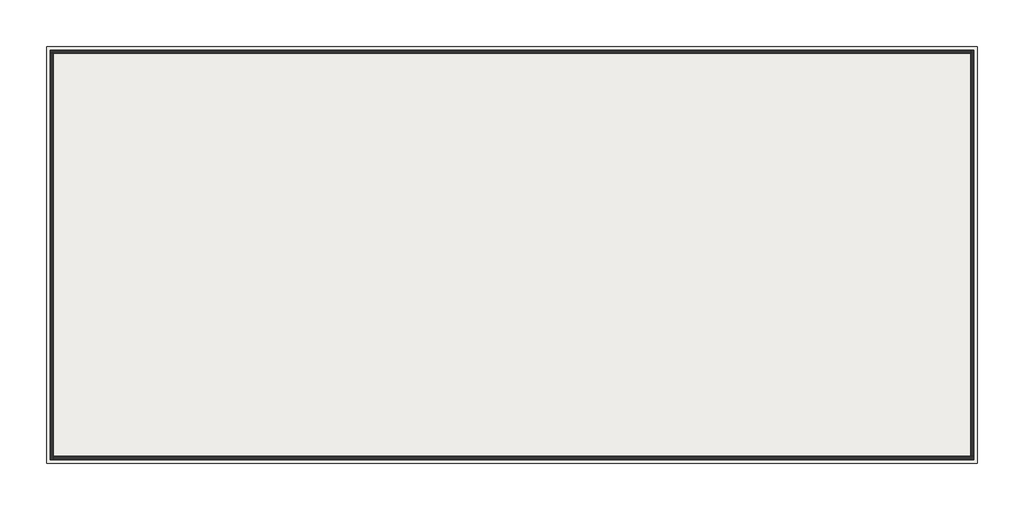
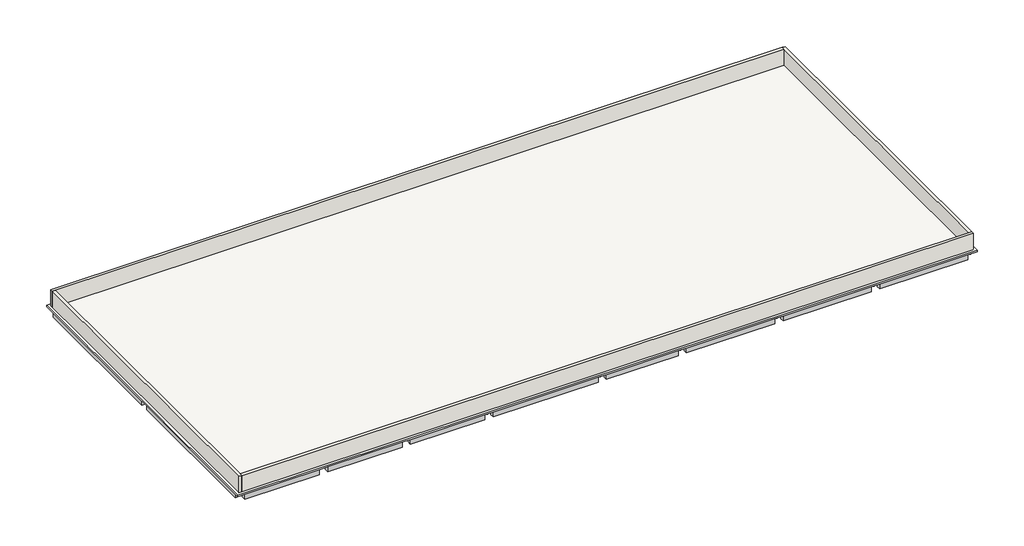
# One storey: 41 beams, 4 walls, 1 roof.
"""IFC4 building model written with IfcOpenShell, lengths in millimetres."""

from ifc_helpers import new_model, si_unit, frame, origin, place, context, project, spatial, polyline, outline, extrude, faceted_brep, element, save

model = new_model("IFC4")

# Units and contexts
model_context = context("Model", 3, world=origin())
ifc_project = project(units=[si_unit("LENGTHUNIT", "METRE", prefix="MILLI")], contexts=[model_context])

# Site, building, storey
site = spatial("IfcSite", under=ifc_project)
building = spatial("IfcBuilding", under=site)
storey = spatial("IfcBuildingStorey", under=building, Name="TOC", Elevation=7649.9618634)

# Beams
placement = place(None, origin())
element("IfcBeam", 1, ObjectType="RC Beam_Rectangular : H_SB_AR_S16_B300xH600", at=placement, inside=storey, context=model_context, shape_type="SweptSolid", body=[
    extrude(outline(polyline([(300.0, 12049.5208589), (300.0, 12349.5208589), (5700.0, 12349.5208589), (5700.0, 12049.5208589), (300.0, 12049.5208589)])), frame((0.0, 0.0, 7049.9618634), z_axis=(0.0, 0.0, 1.0), x_axis=(1.0, 0.0, 0.0)), (0.0, 0.0, 1.0), 499.0),
])
element("IfcBeam", 2, ObjectType="RC Beam_Rectangular : H_SB_AR_S16_B300xH600", at=placement, inside=storey, context=model_context, shape_type="SweptSolid", body=[
    extrude(outline(polyline([(6300.0, 12049.5208589), (6300.0, 12349.5208589), (11700.0, 12349.5208589), (11700.0, 12049.5208589), (6300.0, 12049.5208589)])), frame((0.0, 0.0, 7049.9618634), z_axis=(0.0, 0.0, 1.0), x_axis=(1.0, 0.0, 0.0)), (0.0, 0.0, 1.0), 499.0),
])
element("IfcBeam", 3, ObjectType="RC Beam_Rectangular : H_SB_AR_S16_B300xH600", at=placement, inside=storey, context=model_context, shape_type="SweptSolid", body=[
    extrude(outline(polyline([(12300.0, 12049.5208589), (12300.0, 12349.5208589), (17700.0, 12349.5208589), (17700.0, 12049.5208589), (12300.0, 12049.5208589)])), frame((0.0, 0.0, 7049.9618634), z_axis=(0.0, 0.0, 1.0), x_axis=(1.0, 0.0, 0.0)), (0.0, 0.0, 1.0), 499.0),
])
element("IfcBeam", 4, ObjectType="RC Beam_Rectangular : H_SB_AR_S16_B300xH600", at=placement, inside=storey, context=model_context, shape_type="SweptSolid", body=[
    extrude(outline(polyline([(300.0, 23749.5208589), (300.0, 24049.5208589), (5700.0, 24049.5208589), (5700.0, 23749.5208589), (300.0, 23749.5208589)])), frame((0.0, 0.0, 7049.9618634), z_axis=(0.0, 0.0, 1.0), x_axis=(1.0, 0.0, 0.0)), (0.0, 0.0, 1.0), 499.0),
])
element("IfcBeam", 5, ObjectType="RC Beam_Rectangular : H_SB_AR_S16_B300xH600", at=placement, inside=storey, context=model_context, shape_type="SweptSolid", body=[
    extrude(outline(polyline([(6300.0, 23749.5208589), (6300.0, 24049.5208589), (11700.0, 24049.5208589), (11700.0, 23749.5208589), (6300.0, 23749.5208589)])), frame((0.0, 0.0, 7049.9618634), z_axis=(0.0, 0.0, 1.0), x_axis=(1.0, 0.0, 0.0)), (0.0, 0.0, 1.0), 499.0),
])
element("IfcBeam", 6, ObjectType="RC Beam_Rectangular : H_SB_AR_S16_B300xH600", at=placement, inside=storey, context=model_context, shape_type="SweptSolid", body=[
    extrude(outline(polyline([(12300.0, 23749.5208589), (12300.0, 24049.5208589), (17700.0, 24049.5208589), (17700.0, 23749.5208589), (12300.0, 23749.5208589)])), frame((0.0, 0.0, 7049.9618634), z_axis=(0.0, 0.0, 1.0), x_axis=(1.0, 0.0, 0.0)), (0.0, 0.0, 1.0), 499.0),
])
element("IfcBeam", 7, ObjectType="RC Beam_Rectangular : H_SB_AR_S16_B300xH600", at=placement, inside=storey, context=model_context, shape_type="SweptSolid", body=[
    extrude(outline(polyline([(18300.0, 23749.5208589), (18300.0, 24049.5208589), (25900.0, 24049.5208589), (25900.0, 23749.5208589), (18300.0, 23749.5208589)])), frame((0.0, 0.0, 7049.9618634), z_axis=(0.0, 0.0, 1.0), x_axis=(1.0, 0.0, 0.0)), (0.0, 0.0, 1.0), 499.0),
])
element("IfcBeam", 8, ObjectType="RC Beam_Rectangular : H_SB_AR_S16_B300xH600", at=placement, inside=storey, context=model_context, shape_type="SweptSolid", body=[
    extrude(outline(polyline([(26500.0, 23749.5208589), (26500.0, 24049.5208589), (31700.0, 24049.5208589), (31700.0, 23749.5208589), (26500.0, 23749.5208589)])), frame((0.0, 0.0, 7049.9618634), z_axis=(0.0, 0.0, 1.0), x_axis=(1.0, 0.0, 0.0)), (0.0, 0.0, 1.0), 499.0),
])
element("IfcBeam", 9, ObjectType="RC Beam_Rectangular : H_SB_AR_S16_B300xH600", at=placement, inside=storey, context=model_context, shape_type="SweptSolid", body=[
    extrude(outline(polyline([(32300.0, 23749.5208589), (32300.0, 24049.5208589), (38700.0, 24049.5208589), (38700.0, 23749.5208589), (32300.0, 23749.5208589)])), frame((0.0, 0.0, 7049.9618634), z_axis=(0.0, 0.0, 1.0), x_axis=(1.0, 0.0, 0.0)), (0.0, 0.0, 1.0), 499.0),
])
element("IfcBeam", 10, ObjectType="RC Beam_Rectangular : H_SB_AR_S16_B300xH600", at=placement, inside=storey, context=model_context, shape_type="SweptSolid", body=[
    extrude(outline(polyline([(39300.0, 23749.5208589), (39300.0, 24049.5208589), (45700.0, 24049.5208589), (45700.0, 23749.5208589), (39300.0, 23749.5208589)])), frame((0.0, 0.0, 7049.9618634), z_axis=(0.0, 0.0, 1.0), x_axis=(1.0, 0.0, 0.0)), (0.0, 0.0, 1.0), 499.0),
])
element("IfcBeam", 11, ObjectType="RC Beam_Rectangular : H_SB_AR_S16_B300xH600", at=placement, inside=storey, context=model_context, shape_type="SweptSolid", body=[
    extrude(outline(polyline([(46300.0, 23749.5208589), (46300.0, 24049.5208589), (52700.0, 24049.5208589), (52700.0, 23749.5208589), (46300.0, 23749.5208589)])), frame((0.0, 0.0, 7049.9618634), z_axis=(0.0, 0.0, 1.0), x_axis=(1.0, 0.0, 0.0)), (0.0, 0.0, 1.0), 499.0),
])
element("IfcBeam", 12, ObjectType="RC Beam_Rectangular : H_SB_AR_S16_B300xH600", at=placement, inside=storey, context=model_context, shape_type="SweptSolid", body=[
    extrude(outline(polyline([(26500.0, 8149.5208589), (26500.0, 8449.5208589), (31700.0, 8449.5208589), (31700.0, 8149.5208589), (26500.0, 8149.5208589)])), frame((0.0, 0.0, 7049.9618634), z_axis=(0.0, 0.0, 1.0), x_axis=(1.0, 0.0, 0.0)), (0.0, 0.0, 1.0), 499.0),
])
element("IfcBeam", 13, ObjectType="RC Beam_Rectangular : H_SB_AR_S16_B300xH600", at=placement, inside=storey, context=model_context, shape_type="SweptSolid", body=[
    extrude(outline(polyline([(32300.0, 8149.5208589), (32300.0, 8449.5208589), (38700.0, 8449.5208589), (38700.0, 8149.5208589), (32300.0, 8149.5208589)])), frame((0.0, 0.0, 7049.9618634), z_axis=(0.0, 0.0, 1.0), x_axis=(1.0, 0.0, 0.0)), (0.0, 0.0, 1.0), 499.0),
])
element("IfcBeam", 14, ObjectType="RC Beam_Rectangular : H_SB_AR_S16_B300xH600", at=placement, inside=storey, context=model_context, shape_type="SweptSolid", body=[
    extrude(outline(polyline([(39300.0, 8149.5208589), (39300.0, 8449.5208589), (45700.0, 8449.5208589), (45700.0, 8149.5208589), (39300.0, 8149.5208589)])), frame((0.0, 0.0, 7049.9618634), z_axis=(0.0, 0.0, 1.0), x_axis=(1.0, 0.0, 0.0)), (0.0, 0.0, 1.0), 499.0),
])
element("IfcBeam", 15, ObjectType="RC Beam_Rectangular : H_SB_AR_S16_B300xH600", at=placement, inside=storey, context=model_context, shape_type="SweptSolid", body=[
    extrude(outline(polyline([(46300.0, 8149.5208589), (46300.0, 8449.5208589), (52700.0, 8449.5208589), (52700.0, 8149.5208589), (46300.0, 8149.5208589)])), frame((0.0, 0.0, 7049.9618634), z_axis=(0.0, 0.0, 1.0), x_axis=(1.0, 0.0, 0.0)), (0.0, 0.0, 1.0), 499.0),
])
element("IfcBeam", 16, ObjectType="RC Beam_Rectangular : H_SB_AR_S16_B300xH600", at=placement, inside=storey, context=model_context, shape_type="SweptSolid", body=[
    extrude(outline(polyline([(300.0, 349.5208589), (300.0, 649.5208589), (5700.0, 649.5208589), (5700.0, 349.5208589), (300.0, 349.5208589)])), frame((0.0, 0.0, 7049.9618634), z_axis=(0.0, 0.0, 1.0), x_axis=(1.0, 0.0, 0.0)), (0.0, 0.0, 1.0), 499.0),
])
element("IfcBeam", 17, ObjectType="RC Beam_Rectangular : H_SB_AR_S16_B300xH600", at=placement, inside=storey, context=model_context, shape_type="SweptSolid", body=[
    extrude(outline(polyline([(6300.0, 349.5208589), (6300.0, 649.5208589), (11700.0, 649.5208589), (11700.0, 349.5208589), (6300.0, 349.5208589)])), frame((0.0, 0.0, 7049.9618634), z_axis=(0.0, 0.0, 1.0), x_axis=(1.0, 0.0, 0.0)), (0.0, 0.0, 1.0), 499.0),
])
element("IfcBeam", 18, ObjectType="RC Beam_Rectangular : H_SB_AR_S16_B300xH600", at=placement, inside=storey, context=model_context, shape_type="SweptSolid", body=[
    extrude(outline(polyline([(12300.0, 349.5208589), (12300.0, 649.5208589), (17700.0, 649.5208589), (17700.0, 349.5208589), (12300.0, 349.5208589)])), frame((0.0, 0.0, 7049.9618634), z_axis=(0.0, 0.0, 1.0), x_axis=(1.0, 0.0, 0.0)), (0.0, 0.0, 1.0), 499.0),
])
element("IfcBeam", 19, ObjectType="RC Beam_Rectangular : H_SB_AR_S16_B300xH600", at=placement, inside=storey, context=model_context, shape_type="SweptSolid", body=[
    extrude(outline(polyline([(18300.0, 349.5208589), (18300.0, 649.5208589), (25900.0, 649.5208589), (25900.0, 349.5208589), (18300.0, 349.5208589)])), frame((0.0, 0.0, 7049.9618634), z_axis=(0.0, 0.0, 1.0), x_axis=(1.0, 0.0, 0.0)), (0.0, 0.0, 1.0), 499.0),
])
element("IfcBeam", 20, ObjectType="RC Beam_Rectangular : H_SB_AR_S16_B300xH600", at=placement, inside=storey, context=model_context, shape_type="SweptSolid", body=[
    extrude(outline(polyline([(26500.0, 349.5208589), (26500.0, 649.5208589), (31700.0, 649.5208589), (31700.0, 349.5208589), (26500.0, 349.5208589)])), frame((0.0, 0.0, 7049.9618634), z_axis=(0.0, 0.0, 1.0), x_axis=(1.0, 0.0, 0.0)), (0.0, 0.0, 1.0), 499.0),
])
element("IfcBeam", 21, ObjectType="RC Beam_Rectangular : H_SB_AR_S16_B300xH600", at=placement, inside=storey, context=model_context, shape_type="SweptSolid", body=[
    extrude(outline(polyline([(32300.0, 349.5208589), (32300.0, 649.5208589), (38700.0, 649.5208589), (38700.0, 349.5208589), (32300.0, 349.5208589)])), frame((0.0, 0.0, 7049.9618634), z_axis=(0.0, 0.0, 1.0), x_axis=(1.0, 0.0, 0.0)), (0.0, 0.0, 1.0), 499.0),
])
element("IfcBeam", 22, ObjectType="RC Beam_Rectangular : H_SB_AR_S16_B300xH600", at=placement, inside=storey, context=model_context, shape_type="SweptSolid", body=[
    extrude(outline(polyline([(39300.0, 349.5208589), (39300.0, 649.5208589), (45700.0, 649.5208589), (45700.0, 349.5208589), (39300.0, 349.5208589)])), frame((0.0, 0.0, 7049.9618634), z_axis=(0.0, 0.0, 1.0), x_axis=(1.0, 0.0, 0.0)), (0.0, 0.0, 1.0), 499.0),
])
element("IfcBeam", 23, ObjectType="RC Beam_Rectangular : H_SB_AR_S16_B300xH600", at=placement, inside=storey, context=model_context, shape_type="SweptSolid", body=[
    extrude(outline(polyline([(46300.0, 349.5208589), (46300.0, 649.5208589), (52700.0, 649.5208589), (52700.0, 349.5208589), (46300.0, 349.5208589)])), frame((0.0, 0.0, 7049.9618634), z_axis=(0.0, 0.0, 1.0), x_axis=(1.0, 0.0, 0.0)), (0.0, 0.0, 1.0), 499.0),
])
element("IfcBeam", 24, ObjectType="RC Beam_Rectangular : H_SB_AR_S16_B300xH600", at=placement, inside=storey, context=model_context, shape_type="SweptSolid", body=[
    extrude(outline(polyline([(150.0, 799.5208589), (-150.0, 799.5208589), (-150.0, 11899.5208589), (150.0, 11899.5208589), (150.0, 799.5208589)])), frame((0.0, 0.0, 7049.9618634), z_axis=(0.0, 0.0, 1.0), x_axis=(1.0, 0.0, 0.0)), (0.0, 0.0, 1.0), 499.0),
])
element("IfcBeam", 25, ObjectType="RC Beam_Rectangular : H_SB_AR_S16_B300xH600", at=placement, inside=storey, context=model_context, shape_type="SweptSolid", body=[
    extrude(outline(polyline([(-150.0, 23599.5208589), (150.0, 23599.5208589), (150.0, 12499.5208589), (-150.0, 12499.5208589), (-150.0, 23599.5208589)])), frame((0.0, 0.0, 7049.9618634), z_axis=(0.0, 0.0, 1.0), x_axis=(1.0, 0.0, 0.0)), (0.0, 0.0, 1.0), 499.0),
])
element("IfcBeam", 26, ObjectType="RC Beam_Rectangular : H_SB_AR_S16_B300xH600", at=placement, inside=storey, context=model_context, shape_type="SweptSolid", body=[
    extrude(outline(polyline([(5850.0, 11899.5208589), (6150.0, 11899.5208589), (6150.0, 799.5208589), (5850.0, 799.5208589), (5850.0, 11899.5208589)])), frame((0.0, 0.0, 7049.9618634), z_axis=(0.0, 0.0, 1.0), x_axis=(1.0, 0.0, 0.0)), (0.0, 0.0, 1.0), 499.0),
])
element("IfcBeam", 27, ObjectType="RC Beam_Rectangular : H_SB_AR_S16_B300xH600", at=placement, inside=storey, context=model_context, shape_type="SweptSolid", body=[
    extrude(outline(polyline([(6150.0, 12499.5208589), (5850.0, 12499.5208589), (5850.0, 23599.5208589), (6150.0, 23599.5208589), (6150.0, 12499.5208589)])), frame((0.0, 0.0, 7049.9618634), z_axis=(0.0, 0.0, 1.0), x_axis=(1.0, 0.0, 0.0)), (0.0, 0.0, 1.0), 499.0),
])
element("IfcBeam", 28, ObjectType="RC Beam_Rectangular : H_SB_AR_S16_B300xH600", at=placement, inside=storey, context=model_context, shape_type="SweptSolid", body=[
    extrude(outline(polyline([(11850.0, 11899.5208589), (12150.0, 11899.5208589), (12150.0, 799.5208589), (11850.0, 799.5208589), (11850.0, 11899.5208589)])), frame((0.0, 0.0, 7049.9618634), z_axis=(0.0, 0.0, 1.0), x_axis=(1.0, 0.0, 0.0)), (0.0, 0.0, 1.0), 499.0),
])
element("IfcBeam", 29, ObjectType="RC Beam_Rectangular : H_SB_AR_S16_B300xH600", at=placement, inside=storey, context=model_context, shape_type="SweptSolid", body=[
    extrude(outline(polyline([(12150.0, 12499.5208589), (11850.0, 12499.5208589), (11850.0, 23599.5208589), (12150.0, 23599.5208589), (12150.0, 12499.5208589)])), frame((0.0, 0.0, 7049.9618634), z_axis=(0.0, 0.0, 1.0), x_axis=(1.0, 0.0, 0.0)), (0.0, 0.0, 1.0), 499.0),
])
element("IfcBeam", 30, ObjectType="RC Beam_Rectangular : H_SB_AR_S16_B300xH600", at=placement, inside=storey, context=model_context, shape_type="SweptSolid", body=[
    extrude(outline(polyline([(17850.0, 11899.5208589), (18150.0, 11899.5208589), (18150.0, 799.5208589), (17850.0, 799.5208589), (17850.0, 11899.5208589)])), frame((0.0, 0.0, 7049.9618634), z_axis=(0.0, 0.0, 1.0), x_axis=(1.0, 0.0, 0.0)), (0.0, 0.0, 1.0), 499.0),
])
element("IfcBeam", 31, ObjectType="RC Beam_Rectangular : H_SB_AR_S16_B300xH600", at=placement, inside=storey, context=model_context, shape_type="SweptSolid", body=[
    extrude(outline(polyline([(18150.0, 12499.5208589), (17850.0, 12499.5208589), (17850.0, 23599.5208589), (18150.0, 23599.5208589), (18150.0, 12499.5208589)])), frame((0.0, 0.0, 7049.9618634), z_axis=(0.0, 0.0, 1.0), x_axis=(1.0, 0.0, 0.0)), (0.0, 0.0, 1.0), 499.0),
])
element("IfcBeam", 32, ObjectType="RC Beam_Rectangular : H_SB_AR_S16_B300xH600", at=placement, inside=storey, context=model_context, shape_type="SweptSolid", body=[
    extrude(outline(polyline([(26050.0, 7999.5208589), (26350.0, 7999.5208589), (26350.0, 799.5208589), (26050.0, 799.5208589), (26050.0, 7999.5208589)])), frame((0.0, 0.0, 7049.9618634), z_axis=(0.0, 0.0, 1.0), x_axis=(1.0, 0.0, 0.0)), (0.0, 0.0, 1.0), 499.0),
])
element("IfcBeam", 33, ObjectType="RC Beam_Rectangular : H_SB_AR_S16_B300xH600", at=placement, inside=storey, context=model_context, shape_type="SweptSolid", body=[
    extrude(outline(polyline([(26050.0, 23599.5208589), (26350.0, 23599.5208589), (26350.0, 8599.5208589), (26050.0, 8599.5208589), (26050.0, 23599.5208589)])), frame((0.0, 0.0, 7049.9618634), z_axis=(0.0, 0.0, 1.0), x_axis=(1.0, 0.0, 0.0)), (0.0, 0.0, 1.0), 499.0),
])
element("IfcBeam", 34, ObjectType="RC Beam_Rectangular : H_SB_AR_S16_B300xH600", at=placement, inside=storey, context=model_context, shape_type="SweptSolid", body=[
    extrude(outline(polyline([(31850.0, 7999.5208589), (32150.0, 7999.5208589), (32150.0, 799.5208589), (31850.0, 799.5208589), (31850.0, 7999.5208589)])), frame((0.0, 0.0, 7049.9618634), z_axis=(0.0, 0.0, 1.0), x_axis=(1.0, 0.0, 0.0)), (0.0, 0.0, 1.0), 499.0),
])
element("IfcBeam", 35, ObjectType="RC Beam_Rectangular : H_SB_AR_S16_B300xH600", at=placement, inside=storey, context=model_context, shape_type="SweptSolid", body=[
    extrude(outline(polyline([(31850.0, 23599.5208589), (32150.0, 23599.5208589), (32150.0, 8599.5208589), (31850.0, 8599.5208589), (31850.0, 23599.5208589)])), frame((0.0, 0.0, 7049.9618634), z_axis=(0.0, 0.0, 1.0), x_axis=(1.0, 0.0, 0.0)), (0.0, 0.0, 1.0), 499.0),
])
element("IfcBeam", 36, ObjectType="RC Beam_Rectangular : H_SB_AR_S16_B300xH600", at=placement, inside=storey, context=model_context, shape_type="SweptSolid", body=[
    extrude(outline(polyline([(38850.0, 7999.5208589), (39150.0, 7999.5208589), (39150.0, 799.5208589), (38850.0, 799.5208589), (38850.0, 7999.5208589)])), frame((0.0, 0.0, 7049.9618634), z_axis=(0.0, 0.0, 1.0), x_axis=(1.0, 0.0, 0.0)), (0.0, 0.0, 1.0), 499.0),
])
element("IfcBeam", 37, ObjectType="RC Beam_Rectangular : H_SB_AR_S16_B300xH600", at=placement, inside=storey, context=model_context, shape_type="SweptSolid", body=[
    extrude(outline(polyline([(38850.0, 23599.5208589), (39150.0, 23599.5208589), (39150.0, 8599.5208589), (38850.0, 8599.5208589), (38850.0, 23599.5208589)])), frame((0.0, 0.0, 7049.9618634), z_axis=(0.0, 0.0, 1.0), x_axis=(1.0, 0.0, 0.0)), (0.0, 0.0, 1.0), 499.0),
])
element("IfcBeam", 38, ObjectType="RC Beam_Rectangular : H_SB_AR_S16_B300xH600", at=placement, inside=storey, context=model_context, shape_type="SweptSolid", body=[
    extrude(outline(polyline([(45850.0, 7999.5208589), (46150.0, 7999.5208589), (46150.0, 799.5208589), (45850.0, 799.5208589), (45850.0, 7999.5208589)])), frame((0.0, 0.0, 7049.9618634), z_axis=(0.0, 0.0, 1.0), x_axis=(1.0, 0.0, 0.0)), (0.0, 0.0, 1.0), 499.0),
])
element("IfcBeam", 39, ObjectType="RC Beam_Rectangular : H_SB_AR_S16_B300xH600", at=placement, inside=storey, context=model_context, shape_type="SweptSolid", body=[
    extrude(outline(polyline([(45850.0, 23599.5208589), (46150.0, 23599.5208589), (46150.0, 8599.5208589), (45850.0, 8599.5208589), (45850.0, 23599.5208589)])), frame((0.0, 0.0, 7049.9618634), z_axis=(0.0, 0.0, 1.0), x_axis=(1.0, 0.0, 0.0)), (0.0, 0.0, 1.0), 499.0),
])
element("IfcBeam", 40, ObjectType="RC Beam_Rectangular : H_SB_AR_S16_B300xH600", at=placement, inside=storey, context=model_context, shape_type="SweptSolid", body=[
    extrude(outline(polyline([(53150.0, 799.5208589), (52850.0, 799.5208589), (52850.0, 7999.5208589), (53150.0, 7999.5208589), (53150.0, 799.5208589)])), frame((0.0, 0.0, 7049.9618634), z_axis=(0.0, 0.0, 1.0), x_axis=(1.0, 0.0, 0.0)), (0.0, 0.0, 1.0), 499.0),
])
element("IfcBeam", 41, ObjectType="RC Beam_Rectangular : H_SB_AR_S16_B300xH600", at=placement, inside=storey, context=model_context, shape_type="SweptSolid", body=[
    extrude(outline(polyline([(53150.0, 8599.5208589), (52850.0, 8599.5208589), (52850.0, 23599.5208589), (53150.0, 23599.5208589), (53150.0, 8599.5208589)])), frame((0.0, 0.0, 7049.9618634), z_axis=(0.0, 0.0, 1.0), x_axis=(1.0, 0.0, 0.0)), (0.0, 0.0, 1.0), 499.0),
])

# Roof
element("IfcRoof", 42, ObjectType="H_RF_AR_B06_Memb_XPS_PE_Protective Conc", at=placement, inside=storey, context=model_context, shape_type="Brep", body=[
    faceted_brep([(53300.0, 24199.5208589, 7548.9618634), (53300.0, 23599.5208589, 7548.9618634), (53300.0, 8599.5208589, 7548.9618634), (53300.0, 7999.5208589, 7548.9618634), (53300.0, 799.5208589, 7548.9618634), (53300.0, 199.5208589, 7548.9618634), (52700.0, 199.5208589, 7548.9618634), (46300.0, 199.5208589, 7548.9618634), (45700.0, 199.5208589, 7548.9618634), (39300.0, 199.5208589, 7548.9618634), (38700.0, 199.5208589, 7548.9618634), (32300.0, 199.5208589, 7548.9618634), (31700.0, 199.5208589, 7548.9618634), (26500.0, 199.5208589, 7548.9618634), (25900.0, 199.5208589, 7548.9618634), (18300.0, 199.5208589, 7548.9618634), (17700.0, 199.5208589, 7548.9618634), (12300.0, 199.5208589, 7548.9618634), (11700.0, 199.5208589, 7548.9618634), (6300.0, 199.5208589, 7548.9618634), (5700.0, 199.5208589, 7548.9618634), (300.0, 199.5208589, 7548.9618634), (-300.0, 199.5208589, 7548.9618634), (-300.0, 799.5208589, 7548.9618634), (-300.0, 11899.5208589, 7548.9618634), (-300.0, 12499.5208589, 7548.9618634), (-300.0, 23599.5208589, 7548.9618634), (-300.0, 24199.5208589, 7548.9618634), (300.0, 24199.5208589, 7548.9618634), (5700.0, 24199.5208589, 7548.9618634), (6300.0, 24199.5208589, 7548.9618634), (11700.0, 24199.5208589, 7548.9618634), (12300.0, 24199.5208589, 7548.9618634), (17700.0, 24199.5208589, 7548.9618634), (18300.0, 24199.5208589, 7548.9618634), (25900.0, 24199.5208589, 7548.9618634), (26500.0, 24199.5208589, 7548.9618634), (31700.0, 24199.5208589, 7548.9618634), (32300.0, 24199.5208589, 7548.9618634), (38700.0, 24199.5208589, 7548.9618634), (39300.0, 24199.5208589, 7548.9618634), (45700.0, 24199.5208589, 7548.9618634), (46300.0, 24199.5208589, 7548.9618634), (52700.0, 24199.5208589, 7548.9618634), (53300.0, 199.5208589, 7649.9618634), (53300.0, 24199.5208589, 7649.9618634), (-300.0, 24199.5208589, 7649.9618634), (-300.0, 199.5208589, 7649.9618634)], [[[0, 1, 2, 3, 4, 5, 6, 7, 8, 9, 10, 11, 12, 13, 14, 15, 16, 17, 18, 19, 20, 21, 22, 23, 24, 25, 26, 27, 28, 29, 30, 31, 32, 33, 34, 35, 36, 37, 38, 39, 40, 41, 42, 43]], [[44, 45, 46, 47]], [[45, 44, 5, 4, 3, 2, 1, 0]], [[46, 45, 0, 43, 42, 41, 40, 39, 38, 37, 36, 35, 34, 33, 32, 31, 30, 29, 28, 27]], [[47, 46, 27, 26, 25, 24, 23, 22]], [[44, 47, 22, 21, 20, 19, 18, 17, 16, 15, 14, 13, 12, 11, 10, 9, 8, 7, 6, 5]]]),
])

# Walls
element("IfcWall", 43, ObjectType="H_WA_AR_B02_Ext Wall_RC T200", at=placement, inside=storey, context=model_context, shape_type="Brep", body=[
    faceted_brep([(-100.0, 23799.5208589, 7649.9618634), (100.0, 23799.5208589, 7649.9618634), (52900.0, 23799.5208589, 7649.9618634), (52900.0, 23799.5208589, 8899.9618634), (100.0, 23799.5208589, 8899.9618634), (-100.0, 23799.5208589, 8899.9618634), (-100.0, 23999.5208589, 7649.9618634), (-100.0, 23999.5208589, 8899.9618634), (52900.0, 23999.5208589, 8899.9618634), (52900.0, 23999.5208589, 7649.9618634)], [[[0, 1, 2, 3, 4, 5]], [[6, 7, 8, 9]], [[2, 1, 0, 6, 9]], [[5, 4, 3, 8, 7]], [[0, 5, 7, 6]], [[3, 2, 9, 8]]]),
])
element("IfcWall", 44, ObjectType="H_WA_AR_B02_Ext Wall_RC T200", at=placement, inside=storey, context=model_context, shape_type="Brep", body=[
    faceted_brep([(100.0, 399.5208589, 7649.9618634), (100.0, 599.5208589, 7649.9618634), (100.0, 23799.5208589, 7649.9618634), (100.0, 23799.5208589, 8899.9618634), (100.0, 599.5208589, 8899.9618634), (100.0, 399.5208589, 8899.9618634), (-100.0, 399.5208589, 7649.9618634), (-100.0, 399.5208589, 8899.9618634), (-100.0, 23799.5208589, 8899.9618634), (-100.0, 23799.5208589, 7649.9618634)], [[[0, 1, 2, 3, 4, 5]], [[6, 7, 8, 9]], [[2, 1, 0, 6, 9]], [[5, 4, 3, 8, 7]], [[0, 5, 7, 6]], [[3, 2, 9, 8]]]),
])
element("IfcWall", 45, ObjectType="H_WA_AR_B02_Ext Wall_RC T200", at=placement, inside=storey, context=model_context, shape_type="Brep", body=[
    faceted_brep([(53100.0, 599.5208589, 7649.9618634), (52900.0, 599.5208589, 7649.9618634), (100.0, 599.5208589, 7649.9618634), (100.0, 599.5208589, 8899.9618634), (52900.0, 599.5208589, 8899.9618634), (53100.0, 599.5208589, 8899.9618634), (53100.0, 399.5208589, 7649.9618634), (53100.0, 399.5208589, 8899.9618634), (100.0, 399.5208589, 8899.9618634), (100.0, 399.5208589, 7649.9618634)], [[[0, 1, 2, 3, 4, 5]], [[6, 7, 8, 9]], [[2, 1, 0, 6, 9]], [[5, 4, 3, 8, 7]], [[0, 5, 7, 6]], [[3, 2, 9, 8]]]),
])
element("IfcWall", 46, ObjectType="H_WA_AR_B02_Ext Wall_RC T200", at=placement, inside=storey, context=model_context, shape_type="Brep", body=[
    faceted_brep([(52900.0, 23999.5208589, 7649.9618634), (52900.0, 23799.5208589, 7649.9618634), (52900.0, 599.5208589, 7649.9618634), (52900.0, 599.5208589, 8899.9618634), (52900.0, 23799.5208589, 8899.9618634), (52900.0, 23999.5208589, 8899.9618634), (53100.0, 23999.5208589, 7649.9618634), (53100.0, 23999.5208589, 8899.9618634), (53100.0, 599.5208589, 8899.9618634), (53100.0, 599.5208589, 7649.9618634)], [[[0, 1, 2, 3, 4, 5]], [[6, 7, 8, 9]], [[2, 1, 0, 6, 9]], [[5, 4, 3, 8, 7]], [[0, 5, 7, 6]], [[3, 2, 9, 8]]]),
])

save(model, "model.ifc")

# Revit data of these elements
# Type "RC Beam_Rectangular : H_SB_AR_S16_B300xH600"
#   중앙부 하부근 = ""
#   중앙부 상부근 = ""
#   중앙부 보조근 = ""
#   중앙부 늑근 = ""
#   외단부 하부근 = ""
#   외단부 상부근 = ""
#   외단부 보조근 = ""
#   외단부 늑근 = ""
#   부호 = "TG3"
#   내단부 하부근 = ""
#   내단부 상부근 = ""
#   내단부 보조근 = ""
#   내단부 늑근 = ""
#   ALL 하부근 = "3-D20"
#   ALL 상부근 = "3-D20"
#   ALL 보조근 = ""
#   ALL 늑근 = "2-D10 @120"
#   Width = 300 mm
#   Height = 600 mm
#   Length [instance default] = 1524 mm
#   b = 300 mm
#   h = 600 mm
#   hec_material3 [instance default] = none
#   hec_material2 [instance default] = none
#   hec_material1 [instance default] = none
#   Structural Material [instance default] = none
#   Assembly Code = ""
# Type "H_RF_AR_B06_Memb_XPS_PE_Protective Conc"
#   Layers, outside or top first: 50 mm no material (function 4); 0 mm no material (function 100); 50 mm no material (function 3); 1 mm no material (function 2)
# Type "H_WA_AR_B02_Ext Wall_RC T200"
#   Type Comments = ""
#   Layers, outside or top first: 0 mm no material (function 100); 0 mm no material (function 100); 200 mm no material (function 1); 0 mm no material (function 100); 0 mm no material (function 100); 0 mm no material (function 100)
# Elements 1, 2, 3, 4, 5, 6, 7, 8, 9, 10, 11, 12, 13, 14, 15, 16, 17, 18, 19, 20, 21, 22, 23, 24, 25, 26, 27, 28, 29, 30, 31, 32, 33, 34, 35, 36, 37, 38, 39, 40, 41 (IfcBeam, "RC Beam_Rectangular : H_SB_AR_S16_B300xH600")
#   Comments = ""
#   hec_material3 = none
#   hec_material2 = none
#   hec_material1 = none
#   Structural Material = none
#   Phase Created = New Construction
# Element 42 (IfcRoof, "H_RF_AR_B06_Memb_XPS_PE_Protective Conc")
#   H_Roof Style Name = "Concrete Slab(Slope)+Insulation+Protection Concrete+Waterproofing"
#   H_Roof_Base Material = "Concrete Slab"
#   H_Roof_Finish-1 = "Liquid Waterproofing"
#   H_Roof_Finish-2 = "Rigid Extruded Polystyrene Foam Insulation(XPS)"
#   H_Roof_Finish-3 = "Welded Wire Fabric"
#   H_Roof_Finish-4 = "Protective Concrete w/ Steel Trowel Finish"
#   H_Roof_Finish-5 = "스카이패널 건식복합방수"
#   H_Roof_Style Remark = "* 스카이패널 건식복합방수 : WM 없음"
#   built-in parameter 1001705 = 25.0983 (stored number, unit not read)
#   built-in parameter 1001701 = -0.331365 (stored number, unit not read)
#   built-in parameter 1001710 = 33615
#   H_Roof Style No = RF41
#   Phase Created = New Construction
#   Materials on its faces: "Default Roof"
# Elements 43, 44, 45, 46 (IfcWall, "H_WA_AR_B02_Ext Wall_RC T200")
#   Top Offset = 0 mm
#   Base Offset = 0 mm
#   wall height = 1250 mm
#   Phase Created = New Construction
#   Base Constraint = TOC
#   Top Constraint = TOP
#   Materials on its faces: "Default Wall"
# Materials
#   "Default Roof": class "Miscellaneous", colour RGB 80 80 80, transparency 0
#   "Default Wall": class "Miscellaneous", colour RGB 80 80 80, transparency 0
